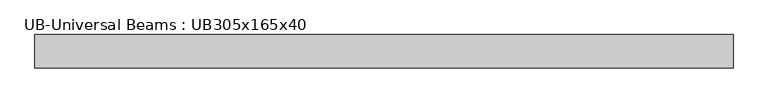
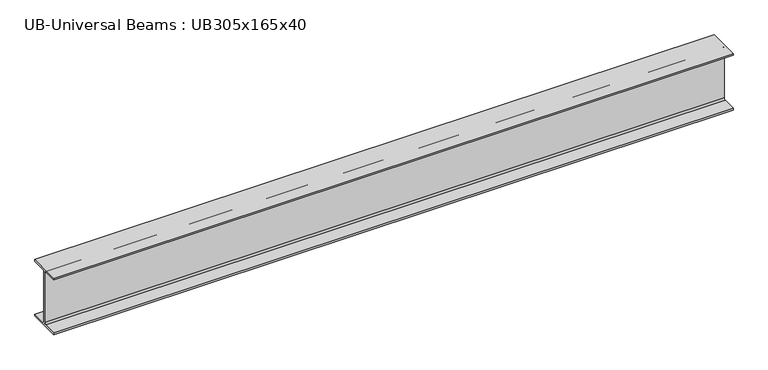
"""IFC4 building model written with IfcOpenShell, lengths in millimetres: beam geometry, UB-Universal Beams : UB305x165x40."""

import ifcopenshell
import ifcopenshell.guid

model = None  # the IFC model being written
_history = None  # IfcOwnerHistory: only IFC2X3 demands one
_inside = {}  # id of a spatial element -> (the spatial element, [elements in it])
_under = {}  # id of a project, library or spatial element -> (it, [spatial elements below it])
_declared = {}  # id of a project -> (the project, [libraries it declares])
_typed = {}  # id of a type object -> (the type object, [elements of that type])
_made_of = {}  # id of a material, layer set ... -> (it, [elements and type objects made of it])


def new_model(schema):
    """Start an empty IFC model of exactly this schema.

    Asked for "IFC4X3", IfcOpenShell would pick the latest addendum, in which some entities
    have other attributes; the version numbers below select the first issue.
    IFC2X3 requires an IfcOwnerHistory on every rooted entity: one is made here for all.
    """
    global model, _history
    if schema == "IFC4X3":
        model = ifcopenshell.file(schema_version=(4, 3, 0, 0))
    else:
        model = ifcopenshell.file(schema=schema)
    _inside.clear()
    _under.clear()
    _declared.clear()
    _typed.clear()
    _made_of.clear()
    _history = None
    if model.schema == "IFC2X3":
        org = make("IfcOrganization", Name="unknown")
        user = make(
            "IfcPersonAndOrganization",
            ThePerson=make("IfcPerson", FamilyName="unknown"),
            TheOrganization=org,
        )
        app = make(
            "IfcApplication",
            ApplicationDeveloper=org,
            Version="unknown",
            ApplicationFullName="unknown",
            ApplicationIdentifier="unknown",
        )
        _history = make(
            "IfcOwnerHistory",
            OwningUser=user,
            OwningApplication=app,
            ChangeAction="ADDED",
            CreationDate=0,
        )
    return model


def make(cls, **values):
    """One entity of the class cls with the attributes given. An attribute that is None is left unset."""
    return model.create_entity(
        cls, **{name: value for name, value in values.items() if value is not None}
    )


def rooted(cls, **values):
    """An entity with a GlobalId (a new one), such as an element, a storey or a relation."""
    return make(cls, GlobalId=ifcopenshell.guid.new(), OwnerHistory=_history, **values)


def si_unit(unit_type, name, prefix=None):
    """IfcSIUnit, for example si_unit("LENGTHUNIT", "METRE", prefix="MILLI")."""
    return make("IfcSIUnit", UnitType=unit_type, Prefix=prefix, Name=name)


def assignment(units):
    """IfcUnitAssignment: the units of a project."""
    return None if units is None else make("IfcUnitAssignment", Units=units)


def point(xyz):
    """IfcCartesianPoint."""
    return None if xyz is None else make("IfcCartesianPoint", Coordinates=xyz)


def direction(xyz):
    """IfcDirection."""
    return None if xyz is None else make("IfcDirection", DirectionRatios=xyz)


def frame(location, z_axis=None, x_axis=None):
    """IfcAxis2Placement3D, a coordinate frame: its origin and axes. An axis left out is left unset."""
    return make(
        "IfcAxis2Placement3D",
        Location=point(location),
        Axis=direction(z_axis),
        RefDirection=direction(x_axis),
    )


def frame_2d(location, x_axis=None):
    """IfcAxis2Placement2D, a coordinate frame in the plane: its origin and x axis."""
    return make(
        "IfcAxis2Placement2D", Location=point(location), RefDirection=direction(x_axis)
    )


def origin():
    """The frame at (0, 0, 0) with its axes left unset."""
    return frame((0.0, 0.0, 0.0))


def place(relative_to, where):
    """IfcLocalPlacement: puts the frame where relative to a parent placement (None: the world)."""
    return make(
        "IfcLocalPlacement", PlacementRelTo=relative_to, RelativePlacement=where
    )


def context(
    kind, dimensions, precision=None, world=None, true_north=None, identifier=None
):
    """IfcGeometricRepresentationContext, for example the 3D "Model" context."""
    return make(
        "IfcGeometricRepresentationContext",
        ContextIdentifier=identifier,
        ContextType=kind,
        CoordinateSpaceDimension=dimensions,
        Precision=precision,
        WorldCoordinateSystem=world,
        TrueNorth=true_north,
    )


def project(units=None, contexts=None):
    """IfcProject with its units and contexts."""
    return rooted(
        "IfcProject",
        Name="project",
        RepresentationContexts=contexts,
        UnitsInContext=assignment(units),
    )


def spatial(cls, under=None, at=None, **own):
    """A site, building, storey or space (cls), placed at a placement, below another one or the project."""
    s = rooted(cls, ObjectPlacement=at, **own)
    if under is not None:
        _under.setdefault(under.id(), (under, []))[1].append(s)
    return s


def polyline(points):
    """IfcPolyline through the points."""
    return make("IfcPolyline", Points=[point(p) for p in points])


def circle_curve(where, radius):
    """IfcCircle in the frame where."""
    return make("IfcCircle", Position=where, Radius=radius)


def trimmed(basis, trim1, trim2, sense, master):
    """IfcTrimmedCurve: the piece of a basis curve between two trims."""
    return make(
        "IfcTrimmedCurve",
        BasisCurve=basis,
        Trim1=trim1,
        Trim2=trim2,
        SenseAgreement=sense,
        MasterRepresentation=master,
    )


def segment(curve, same_sense, transition):
    """IfcCompositeCurveSegment."""
    return make(
        "IfcCompositeCurveSegment",
        Transition=transition,
        SameSense=same_sense,
        ParentCurve=curve,
    )


def composite_curve(segments, self_intersect=None):
    """IfcCompositeCurve: segments joined end to end."""
    return make("IfcCompositeCurve", Segments=segments, SelfIntersect=self_intersect)


def outline(outer, holes=None, kind="AREA"):
    """IfcArbitraryClosedProfileDef: a profile drawn as a closed curve; with holes, ...WithVoids."""
    if holes is None:
        return make("IfcArbitraryClosedProfileDef", ProfileType=kind, OuterCurve=outer)
    return make(
        "IfcArbitraryProfileDefWithVoids",
        ProfileType=kind,
        OuterCurve=outer,
        InnerCurves=holes,
    )


def extrude(swept, where, along, depth):
    """IfcExtrudedAreaSolid: the profile swept, set in the frame where, extruded along a direction by depth."""
    return make(
        "IfcExtrudedAreaSolid",
        SweptArea=swept,
        Position=where,
        ExtrudedDirection=direction(along),
        Depth=depth,
    )


def shape(context_of_items, identifier, shape_type, items):
    """IfcShapeRepresentation: the items that make up one representation, for example the "Body"."""
    return make(
        "IfcShapeRepresentation",
        ContextOfItems=context_of_items,
        RepresentationIdentifier=identifier,
        RepresentationType=shape_type,
        Items=items,
    )


def source(mapping_origin, context_of_items, identifier, shape_type, items):
    """IfcRepresentationMap: a shape defined once, which mapped items show again and again."""
    return make(
        "IfcRepresentationMap",
        MappingOrigin=mapping_origin,
        MappedRepresentation=shape(context_of_items, identifier, shape_type, items),
    )


def transform(
    local_origin,
    x_axis=None,
    y_axis=None,
    z_axis=None,
    scale=None,
    scale2=None,
    scale3=None,
    uniform=True,
):
    """IfcCartesianTransformationOperator3D, or its non-uniform kind. x_axis, y_axis, z_axis: its Axis1, 2, 3."""
    if uniform:
        return make(
            "IfcCartesianTransformationOperator3D",
            Axis1=direction(x_axis),
            Axis2=direction(y_axis),
            LocalOrigin=point(local_origin),
            Scale=scale,
            Axis3=direction(z_axis),
        )
    return make(
        "IfcCartesianTransformationOperator3DnonUniform",
        Axis1=direction(x_axis),
        Axis2=direction(y_axis),
        LocalOrigin=point(local_origin),
        Scale=scale,
        Axis3=direction(z_axis),
        Scale2=scale2,
        Scale3=scale3,
    )


def mapped(mapping_source, mapping_target):
    """IfcMappedItem: shows the shape of a source again, moved by a transform."""
    return make(
        "IfcMappedItem", MappingSource=mapping_source, MappingTarget=mapping_target
    )


def made_of(thing, what):
    """Note that an element or type object is made of a material, layer set ...; save() writes the relation."""
    if what is not None:
        _made_of.setdefault(what.id(), (what, []))[1].append(thing)
    return thing


def element(
    cls,
    number,
    at=None,
    inside=None,
    cuts=None,
    type_object=None,
    material=None,
    context=None,
    identifier="Body",
    shape_type=None,
    held_by="IfcProductDefinitionShape",
    body=None,
    shapes=None,
    **own,
):
    """One element of the class cls, such as IfcWall. Its Tag is "e" and its number.

    at: its placement. inside: the storey or other place that contains it. cuts: it is an
    opening in that element (IfcRelVoidsElement). A single representation is given by context,
    identifier, shape_type and body (its items); several are given by shapes. held_by: the class
    of the entity that holds the representations. save() writes the other relations.
    """
    e = rooted(cls, Tag="e%d" % number, ObjectPlacement=at, **own)
    if body is not None:
        shapes = [shape(context, identifier, shape_type, body)]
    if shapes is not None:
        e.Representation = make(held_by, Representations=shapes)
    if inside is not None:
        _inside.setdefault(inside.id(), (inside, []))[1].append(e)
    if cuts is not None:
        rooted(
            "IfcRelVoidsElement", RelatingBuildingElement=cuts, RelatedOpeningElement=e
        )
    if type_object is not None:
        _typed.setdefault(type_object.id(), (type_object, []))[1].append(e)
    return made_of(e, material)


def aggregate(whole, parts):
    """IfcRelAggregates: a whole, such as a stair, and the parts it consists of."""
    return rooted("IfcRelAggregates", RelatingObject=whole, RelatedObjects=parts)


def save(model, path):
    """Write the relations noted so far, then the file.

    IfcRelAggregates (storeys below a building ...), IfcRelContainedInSpatialStructure (elements
    in a storey), IfcRelDefinesByType, IfcRelAssociatesMaterial and IfcRelDeclares: one each for
    every whole, place, type object, material and project.
    """
    for whole, parts in _under.values():
        aggregate(whole, parts)
    for where, things in _inside.values():
        rooted(
            "IfcRelContainedInSpatialStructure",
            RelatedElements=things,
            RelatingStructure=where,
        )
    for kind, things in _typed.values():
        rooted("IfcRelDefinesByType", RelatedObjects=things, RelatingType=kind)
    for what, things in _made_of.values():
        rooted("IfcRelAssociatesMaterial", RelatedObjects=things, RelatingMaterial=what)
    for by, libraries in _declared.values():
        rooted("IfcRelDeclares", RelatingContext=by, RelatedDefinitions=libraries)
    model.write(path)


def ub_universal_beams_ub305x165x40_daa15f39(model_context):
    return source(origin(), model_context, "Body", "SweptSolid", [
        extrude(outline(composite_curve([segment(polyline([(82.5, -141.5), (82.5, -151.7), (-82.5, -151.7), (-82.5, -141.5), (-11.9, -141.5)]), True, "CONTINUOUS"), segment(trimmed(circle_curve(frame_2d((-11.9, -132.6)), 8.9), [point((-11.9, -141.5))], [point((-3.0, -132.6))], True, "CARTESIAN"), True, "CONTINUOUS"), segment(polyline([(-3.0, -132.6), (-3.0, 132.6)]), True, "CONTINUOUS"), segment(trimmed(circle_curve(frame_2d((-11.9, 132.6)), 8.9), [point((-3.0, 132.6))], [point((-11.9, 141.5))], True, "CARTESIAN"), True, "CONTINUOUS"), segment(polyline([(-11.9, 141.5), (-82.5, 141.5), (-82.5, 151.7), (82.5, 151.7), (82.5, 141.5), (11.9, 141.5)]), True, "CONTINUOUS"), segment(trimmed(circle_curve(frame_2d((11.9, 132.6)), 8.9), [point((11.9, 141.5))], [point((3.0, 132.6))], True, "CARTESIAN"), True, "CONTINUOUS"), segment(polyline([(3.0, 132.6), (3.0, -132.6)]), True, "CONTINUOUS"), segment(trimmed(circle_curve(frame_2d((11.9, -132.6)), 8.9), [point((3.0, -132.6))], [point((11.9, -141.5))], True, "CARTESIAN"), True, "CONTINUOUS"), segment(polyline([(11.9, -141.5), (82.5, -141.5)]), True, "CONTINUOUS")], self_intersect=False)), frame((-1724.05, 0.0, 0.0), z_axis=(1.0, 0.0, 0.0), x_axis=(0.0, 1.0, 0.0)), (0.0, 0.0, 1.0), 3448.1),
    ])


if __name__ == "__main__":
    model = new_model("IFC4")
    model_context = context("Model", 3, world=origin())
    ifc_project = project(units=[si_unit("LENGTHUNIT", "METRE", prefix="MILLI")], contexts=[model_context])
    site = spatial("IfcSite", under=ifc_project)
    building = spatial("IfcBuilding", under=site)
    placement = place(None, origin())
    ub_universal_beams_ub305x165x40_shape = ub_universal_beams_ub305x165x40_daa15f39(model_context)
    element("IfcBeam", 1, ObjectType="UB-Universal Beams : UB305x165x40", at=placement, inside=building, context=model_context, shape_type="MappedRepresentation", body=[
        mapped(ub_universal_beams_ub305x165x40_shape, transform((0.0, 0.0, 0.0), x_axis=(1.0, 0.0, 0.0), y_axis=(0.0, 1.0, 0.0), z_axis=(0.0, 0.0, 1.0))),
    ])
    save(model, "model.ifc")

# Revit data of these elements
# Type "UB-Universal Beams : UB305x165x40"
#   Section Name Key = "UB305X165X40"
#   Width = 16.5 cm
#   Web Thickness = 0.6 cm
#   Web Fillet = 0.89 cm
#   Warping Constant = 164000.0 cm⁶
#   Torsional Moment of Inertia = 14.70 cm⁴
#   Section Area = 51.3 cm²
#   Plastic Modulus weak axis = 142.0 cm³
#   Plastic Modulus strong axis = 623.0 cm³
#   Nominal Weight = 40.2999 kgf/m
#   Moment of Inertia weak axis = 764.00 cm⁴
#   Moment of Inertia strong axis = 8503.00 cm⁴
#   Height = 30.34 cm
#   Flange Thickness = 1.02 cm
#   Elastic Modulus weak axis = 92.6 cm³
#   Elastic Modulus strong axis = 560.0 cm³
#   Centroid Vertical = 15.17 cm
#   Centroid Horizontal = 8.25 cm
#   Bolt Spacing = 9.0 cm
#   Length [instance default] = 1500 mm
#   Structural Material [instance default] = Metal - Steel 43-275
#   Type Comments = ""
#   Assembly Code = ""
# Element 1 (IfcBeam, "UB-Universal Beams : UB305x165x40")
#   Materials on its faces: "Metal - Steel 43-275"
# Materials
#   "Metal - Steel 43-275": class "Metal", colour RGB 247 247 247, transparency 0, Cost = 0
